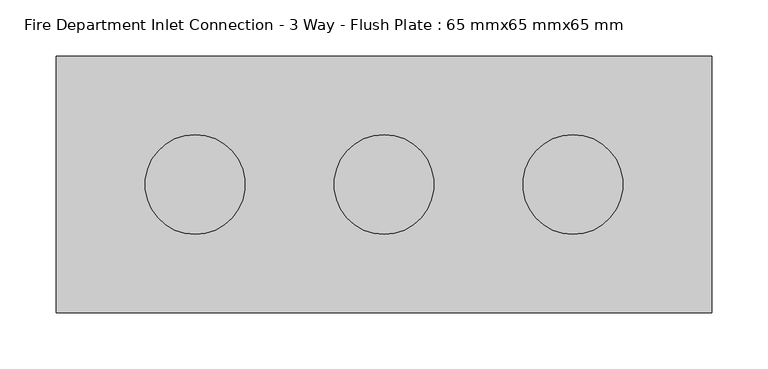
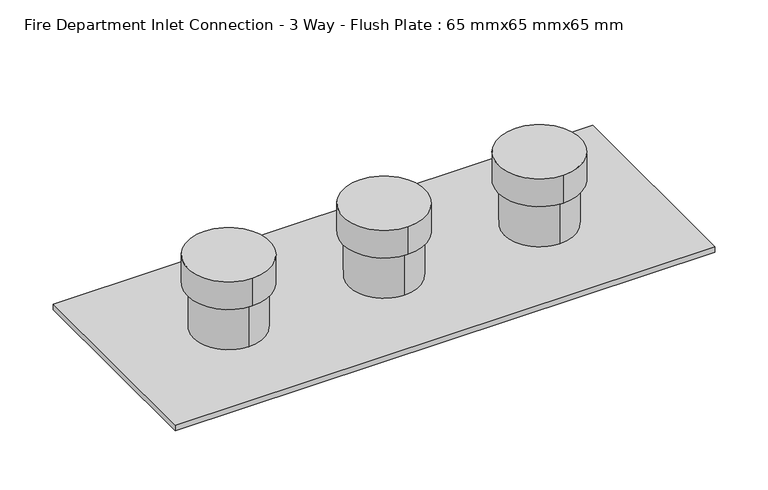
"""IFC4 building model written with IfcOpenShell, lengths in millimetres: proxy geometry, Fire Department Inlet Connection - 3 Way - Flush Plate : 65 mmx65 mmx65 mm."""

from ifc_helpers import new_model, si_unit, point, frame, frame_2d, origin, origin_with_axes, origin_2d, place, context, project, spatial, polyline, circle_curve, trimmed, segment, composite_curve, outline, extrude, source, transform, mapped, element, save
from ifc_brep_helpers import plane_surface, cylinder_surface, advanced_brep


def fire_department_inlet_connection_3_way_flush_plate_65_mmx65_f46b15d6(model_context):
    return source(origin(), model_context, "Body", "SolidModel", [
        extrude(outline(polyline([(292.1, 114.3), (292.1, -114.3), (-292.1, -114.3), (-292.1, 114.3), (292.1, 114.3)])), frame((0.0, 0.0, 6.35), z_axis=(0.0, 0.0, 1.0), x_axis=(1.0, 0.0, 0.0)), (0.0, 0.0, 1.0), 6.35),
        advanced_brep(
        [(168.275, 44.45, 95.25), (168.275, -44.45, 95.25), (168.275, 44.45, 63.5), (168.275, -44.45, 63.5), (168.275, 38.1, 63.5), (168.275, -38.1, 63.5), (168.275, 38.1, 12.7), (168.275, -38.1, 12.7)],
        [
            (0, 1, circle_curve(frame((168.275, 0.0, 95.25), z_axis=(0.0, 0.0, 1.0), x_axis=(0.0, -1.0, 0.0)), 44.45)),
            (1, 0, circle_curve(frame((168.275, 0.0, 95.25), z_axis=(0.0, 0.0, 1.0), x_axis=(0.0, -1.0, 0.0)), 44.45)),
            (2, 3, circle_curve(frame((168.275, 0.0, 63.5), z_axis=(0.0, 0.0, -1.0), x_axis=(0.0, -1.0, 0.0)), 44.45)),
            (3, 2, circle_curve(frame((168.275, 0.0, 63.5), z_axis=(0.0, 0.0, -1.0), x_axis=(0.0, -1.0, 0.0)), 44.45)),
            (4, 5, circle_curve(frame((168.275, 0.0, 63.5), z_axis=(0.0, 0.0, 1.0), x_axis=(0.0, -1.0, 0.0)), 38.1)),
            (5, 4, circle_curve(frame((168.275, 0.0, 63.5), z_axis=(0.0, 0.0, 1.0), x_axis=(0.0, -1.0, 0.0)), 38.1)),
            (0, 2),
            (3, 1),
            (6, 7, circle_curve(frame((168.275, 0.0, 12.7), z_axis=(0.0, 0.0, -1.0), x_axis=(0.0, -1.0, 0.0)), 38.1)),
            (7, 6, circle_curve(frame((168.275, 0.0, 12.7), z_axis=(0.0, 0.0, -1.0), x_axis=(0.0, -1.0, 0.0)), 38.1)),
            (7, 5),
            (4, 6),
        ],
        [
            plane_surface(frame((168.275, -44.45, 95.25), z_axis=(0.0, 0.0, 1.0), x_axis=(1.0, 0.0, 0.0))),
            plane_surface(frame((168.275, -44.45, 63.5), z_axis=(0.0, 0.0, -1.0), x_axis=(-1.0, 0.0, 0.0))),
            cylinder_surface(frame((168.275, 0.0, 63.5), z_axis=(0.0, 0.0, 1.0), x_axis=(0.0, -1.0, 0.0)), 44.45),
            plane_surface(frame((168.275, -38.1, 12.7), z_axis=(0.0, 0.0, -1.0), x_axis=(-1.0, 0.0, 0.0))),
            cylinder_surface(frame((168.275, 0.0, 12.7), z_axis=(0.0, 0.0, 1.0), x_axis=(0.0, -1.0, 0.0)), 38.1),
        ],
        [
            (0, [[1, 2]]),
            (1, [[3, 4], [5, 6]]),
            (2, [[-1, 7, -4, 8]]),
            (2, [[-2, -8, -3, -7]]),
            (3, [[9, 10]]),
            (4, [[-10, 11, -5, 12]]),
            (4, [[-9, -12, -6, -11]]),
        ],
    ),
        advanced_brep(
        [(0.0, 44.45, 95.25), (0.0, -44.45, 95.25), (0.0, 44.45, 63.5), (0.0, -44.45, 63.5), (0.0, 38.1, 63.5), (0.0, -38.1, 63.5), (0.0, 38.1, 12.7), (0.0, -38.1, 12.7)],
        [
            (0, 1, circle_curve(frame((0.0, 0.0, 95.25), z_axis=(0.0, 0.0, 1.0), x_axis=(0.0, -1.0, 0.0)), 44.45)),
            (1, 0, circle_curve(frame((0.0, 0.0, 95.25), z_axis=(0.0, 0.0, 1.0), x_axis=(0.0, -1.0, 0.0)), 44.45)),
            (2, 3, circle_curve(frame((0.0, 0.0, 63.5), z_axis=(0.0, 0.0, -1.0), x_axis=(0.0, -1.0, 0.0)), 44.45)),
            (3, 2, circle_curve(frame((0.0, 0.0, 63.5), z_axis=(0.0, 0.0, -1.0), x_axis=(0.0, -1.0, 0.0)), 44.45)),
            (4, 5, circle_curve(frame((0.0, 0.0, 63.5), z_axis=(0.0, 0.0, 1.0), x_axis=(0.0, -1.0, 0.0)), 38.1)),
            (5, 4, circle_curve(frame((0.0, 0.0, 63.5), z_axis=(0.0, 0.0, 1.0), x_axis=(0.0, -1.0, 0.0)), 38.1)),
            (0, 2),
            (3, 1),
            (6, 7, circle_curve(frame((0.0, 0.0, 12.7), z_axis=(0.0, 0.0, -1.0), x_axis=(0.0, -1.0, 0.0)), 38.1)),
            (7, 6, circle_curve(frame((0.0, 0.0, 12.7), z_axis=(0.0, 0.0, -1.0), x_axis=(0.0, -1.0, 0.0)), 38.1)),
            (7, 5),
            (4, 6),
        ],
        [
            plane_surface(frame((168.275, -44.45, 95.25), z_axis=(0.0, 0.0, 1.0), x_axis=(1.0, 0.0, 0.0))),
            plane_surface(frame((168.275, -44.45, 63.5), z_axis=(0.0, 0.0, -1.0), x_axis=(-1.0, 0.0, 0.0))),
            cylinder_surface(frame((0.0, 0.0, 0.0), z_axis=(0.0, 0.0, 1.0), x_axis=(0.0, -1.0, 0.0)), 44.45),
            plane_surface(frame((168.275, -38.1, 12.7), z_axis=(0.0, 0.0, -1.0), x_axis=(-1.0, 0.0, 0.0))),
            cylinder_surface(frame((0.0, 0.0, 0.0), z_axis=(0.0, 0.0, 1.0), x_axis=(0.0, -1.0, 0.0)), 38.1),
        ],
        [
            (0, [[1, 2]]),
            (1, [[3, 4], [5, 6]]),
            (2, [[-1, 7, -4, 8]]),
            (2, [[-2, -8, -3, -7]]),
            (3, [[9, 10]]),
            (4, [[-10, 11, -5, 12]]),
            (4, [[-9, -12, -6, -11]]),
        ],
    ),
        advanced_brep(
        [(-168.275, 44.45, 95.25), (-168.275, -44.45, 95.25), (-168.275, 44.45, 63.5), (-168.275, -44.45, 63.5), (-168.275, 38.1, 63.5), (-168.275, -38.1, 63.5), (-168.275, 38.1, 12.7), (-168.275, -38.1, 12.7)],
        [
            (0, 1, circle_curve(frame((-168.275, 0.0, 95.25), z_axis=(0.0, 0.0, 1.0), x_axis=(0.0, -1.0, 0.0)), 44.45)),
            (1, 0, circle_curve(frame((-168.275, 0.0, 95.25), z_axis=(0.0, 0.0, 1.0), x_axis=(0.0, -1.0, 0.0)), 44.45)),
            (2, 3, circle_curve(frame((-168.275, 0.0, 63.5), z_axis=(0.0, 0.0, -1.0), x_axis=(0.0, -1.0, 0.0)), 44.45)),
            (3, 2, circle_curve(frame((-168.275, 0.0, 63.5), z_axis=(0.0, 0.0, -1.0), x_axis=(0.0, -1.0, 0.0)), 44.45)),
            (4, 5, circle_curve(frame((-168.275, 0.0, 63.5), z_axis=(0.0, 0.0, 1.0), x_axis=(0.0, -1.0, 0.0)), 38.1)),
            (5, 4, circle_curve(frame((-168.275, 0.0, 63.5), z_axis=(0.0, 0.0, 1.0), x_axis=(0.0, -1.0, 0.0)), 38.1)),
            (0, 2),
            (3, 1),
            (6, 7, circle_curve(frame((-168.275, 0.0, 12.7), z_axis=(0.0, 0.0, -1.0), x_axis=(0.0, -1.0, 0.0)), 38.1)),
            (7, 6, circle_curve(frame((-168.275, 0.0, 12.7), z_axis=(0.0, 0.0, -1.0), x_axis=(0.0, -1.0, 0.0)), 38.1)),
            (7, 5),
            (4, 6),
        ],
        [
            plane_surface(frame((168.275, -44.45, 95.25), z_axis=(0.0, 0.0, 1.0), x_axis=(1.0, 0.0, 0.0))),
            plane_surface(frame((168.275, -44.45, 63.5), z_axis=(0.0, 0.0, -1.0), x_axis=(-1.0, 0.0, 0.0))),
            cylinder_surface(frame((-168.275, 0.0, 0.0), z_axis=(0.0, 0.0, 1.0), x_axis=(0.0, -1.0, 0.0)), 44.45),
            plane_surface(frame((168.275, -38.1, 12.7), z_axis=(0.0, 0.0, -1.0), x_axis=(-1.0, 0.0, 0.0))),
            cylinder_surface(frame((-168.275, 0.0, 0.0), z_axis=(0.0, 0.0, 1.0), x_axis=(0.0, -1.0, 0.0)), 38.1),
        ],
        [
            (0, [[1, 2]]),
            (1, [[3, 4], [5, 6]]),
            (2, [[-1, 7, -4, 8]]),
            (2, [[-2, -8, -3, -7]]),
            (3, [[9, 10]]),
            (4, [[-10, 11, -5, 12]]),
            (4, [[-9, -12, -6, -11]]),
        ],
    ),
        extrude(outline(composite_curve([segment(trimmed(circle_curve(frame_2d((168.275, 0.0)), 50.8), [point((168.275, 50.8))], [point((168.275, -50.8))], False, "CARTESIAN"), True, "CONTINUOUS"), segment(trimmed(circle_curve(frame_2d((168.275, 0.0)), 50.8), [point((168.275, -50.8))], [point((168.275, 50.8))], False, "CARTESIAN"), True, "CONTINUOUS")], self_intersect=False)), origin_with_axes(), (0.0, 0.0, 1.0), 6.35),
        extrude(outline(composite_curve([segment(trimmed(circle_curve(origin_2d(), 50.8), [point((0.0, 50.8))], [point((0.0, -50.8))], False, "CARTESIAN"), True, "CONTINUOUS"), segment(trimmed(circle_curve(origin_2d(), 50.8), [point((0.0, -50.8))], [point((0.0, 50.8))], False, "CARTESIAN"), True, "CONTINUOUS")], self_intersect=False)), origin_with_axes(), (0.0, 0.0, 1.0), 6.35),
        extrude(outline(composite_curve([segment(trimmed(circle_curve(frame_2d((-168.275, 0.0)), 50.8), [point((-168.275, 50.8))], [point((-168.275, -50.8))], False, "CARTESIAN"), True, "CONTINUOUS"), segment(trimmed(circle_curve(frame_2d((-168.275, 0.0)), 50.8), [point((-168.275, -50.8))], [point((-168.275, 50.8))], False, "CARTESIAN"), True, "CONTINUOUS")], self_intersect=False)), origin_with_axes(), (0.0, 0.0, 1.0), 6.35),
    ])


if __name__ == "__main__":
    model = new_model("IFC4")
    model_context = context("Model", 3, world=origin())
    ifc_project = project(units=[si_unit("LENGTHUNIT", "METRE", prefix="MILLI")], contexts=[model_context])
    site = spatial("IfcSite", under=ifc_project)
    building = spatial("IfcBuilding", under=site)
    placement = place(None, origin())
    fire_department_inlet_connection_3_way_flush_plate_65_mmx65_shape = fire_department_inlet_connection_3_way_flush_plate_65_mmx65_f46b15d6(model_context)
    element("IfcBuildingElementProxy", 1, Name="Fire Department Inlet Connection - 3 Way - Flush Plate : 65 mmx65 mmx65 mm", ObjectType="Fire Department Inlet Connection - 3 Way - Flush Plate : 65 mmx65 mmx65 mm", at=placement, inside=building, context=model_context, shape_type="MappedRepresentation", body=[
        mapped(fire_department_inlet_connection_3_way_flush_plate_65_mmx65_shape, transform((0.0, 0.0, 0.0), x_axis=(1.0, 0.0, 0.0), y_axis=(0.0, 1.0, 0.0), z_axis=(0.0, 0.0, 1.0))),
    ])
    save(model, "model.ifc")

# Revit data of these elements
# Project information
#   Sheet x = "1"
#   Sheet Total = "4"
#   COBie.CreatedBy = "info@mma.ie"
#   COBie.CreatedOn = "2017-07-04T11:33:08"
#   COBie.Facility.Category = "11-16 27 14 : Mixed-Gender Dormitory"
#   COBie.Facility.ProjectName = "East Dormitory"
#   COBie.Facility.SiteName = "East Healey Street, Champaign, Illinois, USA"
#   COBie.Facility.LinearUnits = "Millimeters"
#   COBie.Facility.AreaUnits = "Square Meters"
#   COBie.Facility.VolumeUnits = "Cubic Meters"
#   COBie.Facility.CurrencyUnit = "None"
#   COBie.Facility.AreaMeasurement = "Revit Default Area Calculation Method"
#   COBie.Facility.Description = "Two Storey Luxury Dormitory"
#   COBie.Facility.ProjectDescription = "One of Four Dormitories on the E.Healey Site"
#   COBie.Facility.SiteDescription = "Four Dormitories Project Site"
#   COBie.Facility.Phase = "60% Design Submission"
#   Classification.Facility.Description = "Mixed-Gender Dormitory"
#   Classification.Facility.Number = "11-16 27 14"
#   Project Issue Date = "Issue Date"
#   Project Status = "Final Issue"
#   Client Name = "Prairie Sky Consulting"
#   Project Address = "East Healey Street, \nChampaign, \nIllinois, \nUSA"
#   Project Name = "Four Dormitory Complex"
#   Project Number = "East Dormitory"
# Type "Fire Department Inlet Connection - 3 Way - Flush Plate : 65 mmx65 mmx65 mm"
#   Type Mark = "Fire Department Inlet Connection - 3 Way - Flush Plate"
#   COBie.Type.CreatedBy = "info@mma.ie"
#   COBie.Type.CreatedOn = "2017-07-04T11:33:08"
#   COBie.Type.Name = "Fire Department Inlet Connection - 3 Way - Flush Plate"
#   COBie.Type.Category = "23-29 25 15 : Fire Hose Equipment"
#   COBie.Type.Description = "Fire Department Inlet Connection - 3 Way - Flush Plate_65 mmx65 mmx65 mm"
#   COBie.Type.AssetType = "Fixed"
#   COBie.Type.Manufacturer = ""
#   COBie.Type.ModelNumber = ""
#   COBie.Type.ModelReference = "21 11 19.A"
#   Classification.OmniClass.23.Number = "23-29 25 15"
#   Classification.OmniClass.23.Description = "Fire Hose Equipment"
#   Keynote = "21 11 19.A"
#   F.I.-Material = "Polished Brass Plate"
#   F.I.-Inlet = ""
#   F.I. No. of Inlets = "3"
#   COBie.Type.ReplacementCost = 0
#   Nominal Radius = 32.5 mm
#   Nominal Diameter = 65 mm
#   F.I. Inlet = 88.9 mm
#   Default Elevation = 700 mm
#   COBie.Type = yes
#   Inlet Connection Plate Material = Polished Brass
# Element 1 (IfcBuildingElementProxy, "Fire Department Inlet Connection - 3 Way - Flush Plate : 65 mmx65 mmx65 mm")
#   Materials on its faces: "Polished Brass"
# Materials
#   "Polished Brass": class "Plastic", colour RGB 120 120 120, transparency 0, Description = "Acrylonitrile butadiene styrene", Cost = 0
